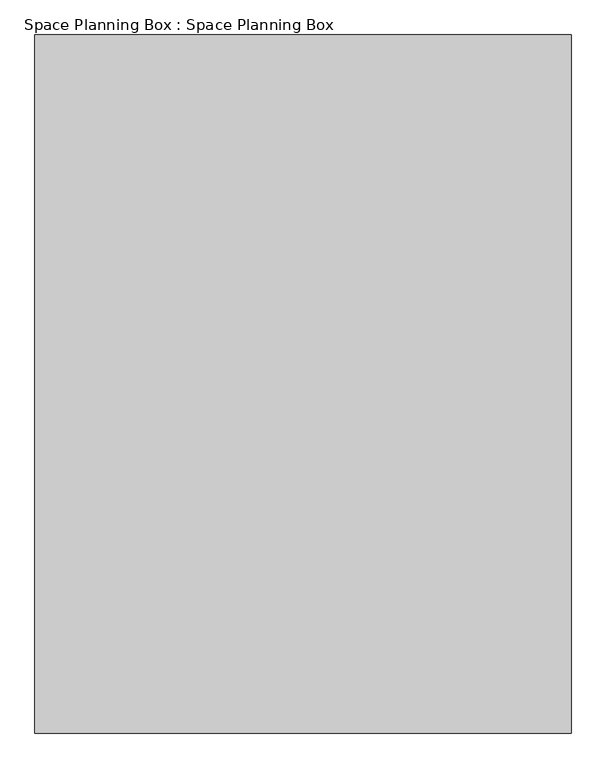
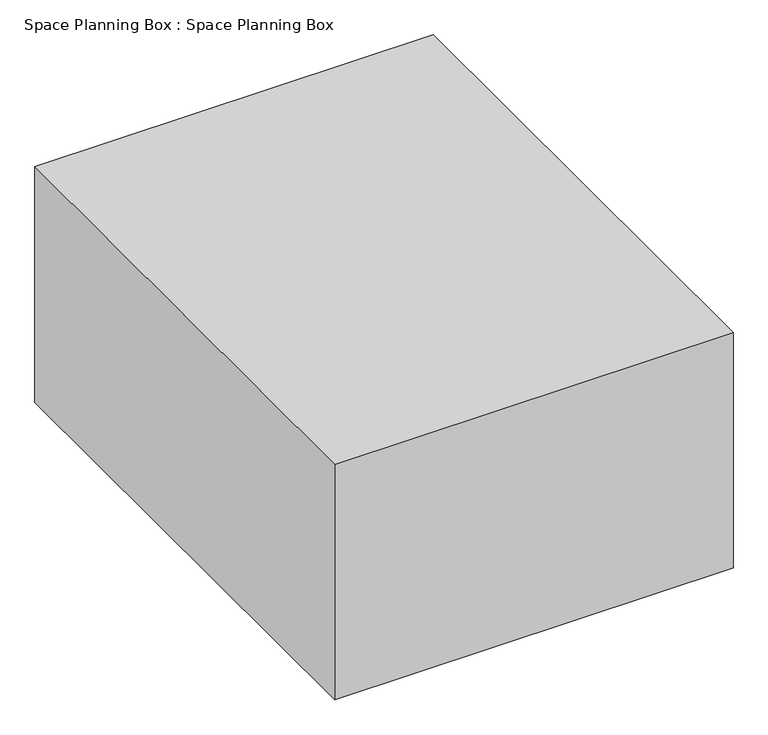
"""IFC4 building model written with IfcOpenShell, lengths in millimetres: proxy geometry, Space Planning Box : Space Planning Box."""

from ifc_helpers import new_model, si_unit, origin, origin_with_axes, place, context, project, spatial, polyline, outline, extrude, source, transform, mapped, element, save


def space_planning_box_space_planning_box_72d488a7(model_context):
    return source(origin(), model_context, "Body", "SweptSolid", [
        extrude(outline(polyline([(4800.0, 6250.0), (4800.0, -6250.0), (-4800.0, -6250.0), (-4800.0, 6250.0), (4800.0, 6250.0)])), origin_with_axes(), (0.0, 0.0, 1.0), 6000.0),
    ])


if __name__ == "__main__":
    model = new_model("IFC4")
    model_context = context("Model", 3, world=origin())
    ifc_project = project(units=[si_unit("LENGTHUNIT", "METRE", prefix="MILLI")], contexts=[model_context])
    site = spatial("IfcSite", under=ifc_project)
    building = spatial("IfcBuilding", under=site)
    placement = place(None, origin())
    space_planning_box_space_planning_box_shape = space_planning_box_space_planning_box_72d488a7(model_context)
    element("IfcBuildingElementProxy", 1, Name="Space Planning Box : Space Planning Box", ObjectType="Space Planning Box : Space Planning Box", at=placement, inside=building, context=model_context, shape_type="MappedRepresentation", body=[
        mapped(space_planning_box_space_planning_box_shape, transform((0.0, 0.0, 0.0), x_axis=(1.0, 0.0, 0.0), y_axis=(0.0, 1.0, 0.0), z_axis=(0.0, 0.0, 1.0))),
    ])
    save(model, "model.ifc")

# Revit data of these elements
# Type "Space Planning Box : Space Planning Box"
#   Type Comments = "..."
#   Room Name [instance default] = "?"
#   Assembly Code = "..."
#   Width [instance default] = 1524 mm
#   Program Area [instance default] = 0 m²
#   Length [instance default] = 1524 mm
#   Height [instance default] = 1524 mm
#   Area [instance default] = 2.32258 m²
#   Fill Color [instance default] = Cyan
#   Default Elevation = 0
# Element 1 (IfcBuildingElementProxy, "Space Planning Box : Space Planning Box")
#   Room Name = "Engineer Room"
#   Width = 9600 mm
#   Program Area = 120 m²
#   Length = 12500 mm
#   Height = 6000 mm
#   Area = 120 m²
#   Fill Color = Lime
#   Materials on its faces: "Lime"
# Materials
#   "Cyan": class "Generic", colour RGB 0 255 255, transparency 0.2, Cost = 0
#   "Lime": class "Generic", colour RGB 0 255 0, transparency 0.2, Cost = 0
